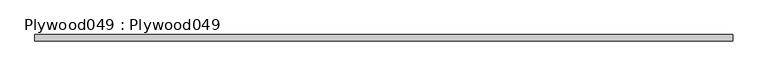
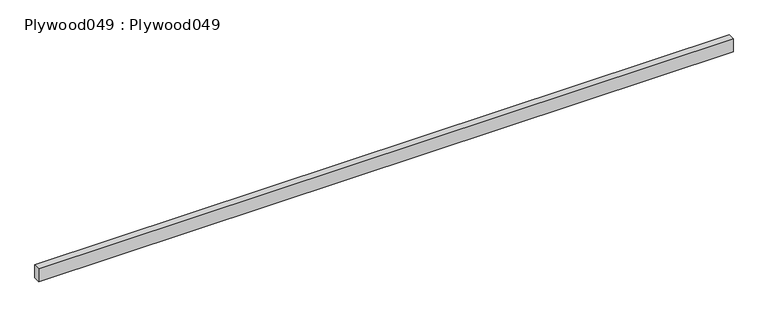
"""IFC4 building model written with IfcOpenShell, lengths in millimetres: proxy geometry, Plywood049 : Plywood049."""

from ifc_helpers import new_model, si_unit, frame, origin, place, context, project, spatial, polyline, outline, extrude, source, transform, mapped, element, save


def plywood049_plywood049_d2740341(model_context):
    return source(origin(), model_context, "Body", "SweptSolid", [
        extrude(outline(polyline([(14383.0178845, -4389.9279008), (14383.0178845, -4408.6354617), (12383.0178845, -4408.6354617), (12383.0178845, -4389.9279008), (14383.0178845, -4389.9279008)])), frame((0.0, 0.0, 42601.896), z_axis=(0.0, 0.0, 1.0), x_axis=(1.0, 0.0, 0.0)), (0.0, 0.0, 1.0), 39.7172813),
    ])


if __name__ == "__main__":
    model = new_model("IFC4")
    model_context = context("Model", 3, world=origin())
    ifc_project = project(units=[si_unit("LENGTHUNIT", "METRE", prefix="MILLI")], contexts=[model_context])
    site = spatial("IfcSite", under=ifc_project)
    building = spatial("IfcBuilding", under=site)
    placement = place(None, origin())
    plywood049_plywood049_shape = plywood049_plywood049_d2740341(model_context)
    element("IfcBuildingElementProxy", 1, Name="Plywood049 : Plywood049", ObjectType="Plywood049 : Plywood049", at=placement, inside=building, context=model_context, shape_type="MappedRepresentation", body=[
        mapped(plywood049_plywood049_shape, transform((0.0, 0.0, 0.0), x_axis=(1.0, 0.0, 0.0), y_axis=(0.0, 1.0, 0.0), z_axis=(0.0, 0.0, 1.0))),
    ])
    save(model, "model.ifc")

# Revit data of these elements
# Type "Plywood049 : Plywood049"
#   NameOverride = "Plywood049"
# Element 1 (IfcBuildingElementProxy, "Plywood049 : Plywood049")
#   Materials on its faces: "CDX PLYWOOD -  SEE STRUCTURAL DWGS"
# Materials
#   "CDX PLYWOOD -  SEE STRUCTURAL DWGS": class "Unassigned", colour RGB 177 130 114, transparency 0, Cost = 0
